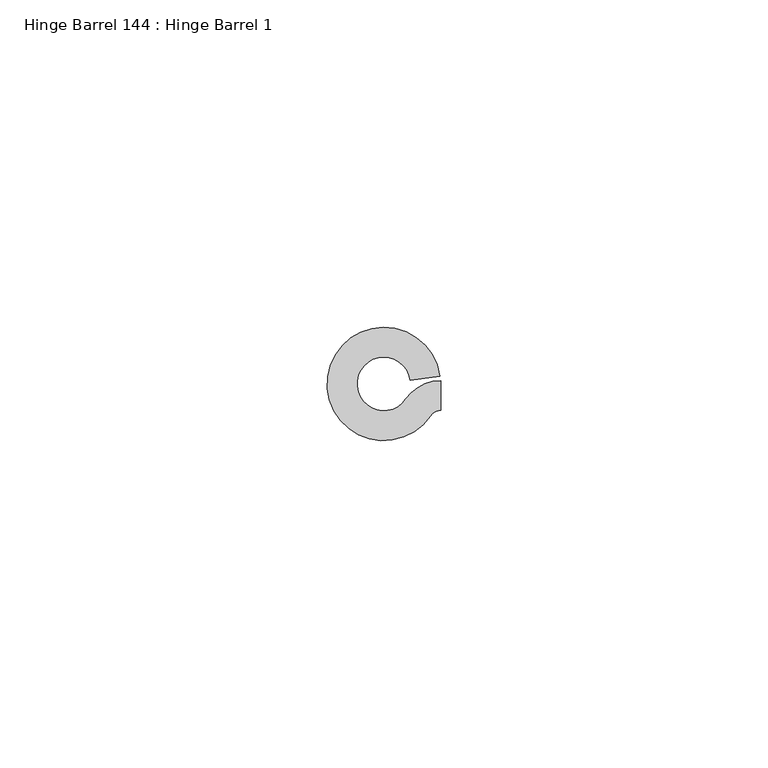
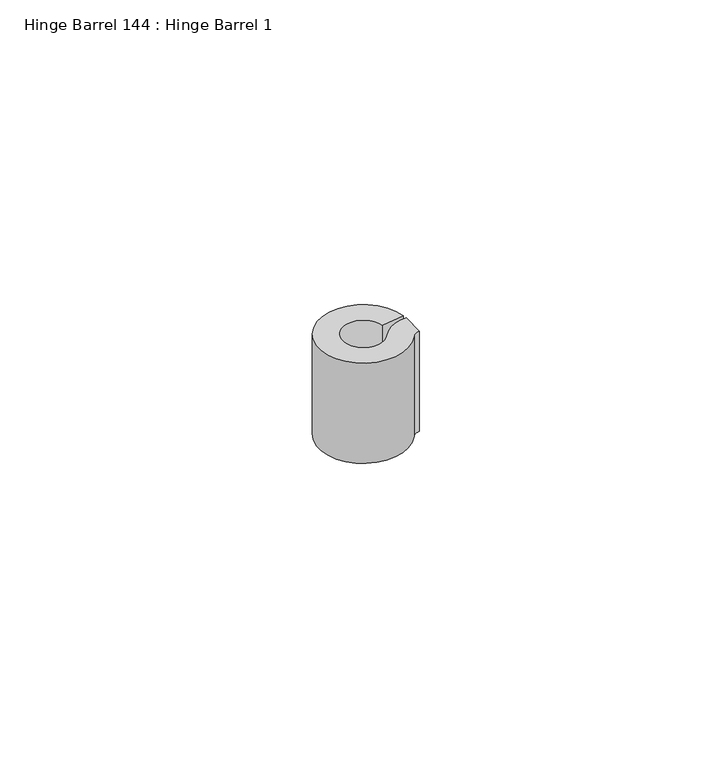
"""IFC4 building model written with IfcOpenShell, lengths in millimetres: proxy geometry, Hinge Barrel 144 : Hinge Barrel 1."""

import ifcopenshell
import ifcopenshell.guid

model = None  # the IFC model being written
_history = None  # IfcOwnerHistory: only IFC2X3 demands one
_inside = {}  # id of a spatial element -> (the spatial element, [elements in it])
_under = {}  # id of a project, library or spatial element -> (it, [spatial elements below it])
_declared = {}  # id of a project -> (the project, [libraries it declares])
_typed = {}  # id of a type object -> (the type object, [elements of that type])
_made_of = {}  # id of a material, layer set ... -> (it, [elements and type objects made of it])


def new_model(schema):
    """Start an empty IFC model of exactly this schema.

    Asked for "IFC4X3", IfcOpenShell would pick the latest addendum, in which some entities
    have other attributes; the version numbers below select the first issue.
    IFC2X3 requires an IfcOwnerHistory on every rooted entity: one is made here for all.
    """
    global model, _history
    if schema == "IFC4X3":
        model = ifcopenshell.file(schema_version=(4, 3, 0, 0))
    else:
        model = ifcopenshell.file(schema=schema)
    _inside.clear()
    _under.clear()
    _declared.clear()
    _typed.clear()
    _made_of.clear()
    _history = None
    if model.schema == "IFC2X3":
        org = make("IfcOrganization", Name="unknown")
        user = make(
            "IfcPersonAndOrganization",
            ThePerson=make("IfcPerson", FamilyName="unknown"),
            TheOrganization=org,
        )
        app = make(
            "IfcApplication",
            ApplicationDeveloper=org,
            Version="unknown",
            ApplicationFullName="unknown",
            ApplicationIdentifier="unknown",
        )
        _history = make(
            "IfcOwnerHistory",
            OwningUser=user,
            OwningApplication=app,
            ChangeAction="ADDED",
            CreationDate=0,
        )
    return model


def make(cls, **values):
    """One entity of the class cls with the attributes given. An attribute that is None is left unset."""
    return model.create_entity(
        cls, **{name: value for name, value in values.items() if value is not None}
    )


def rooted(cls, **values):
    """An entity with a GlobalId (a new one), such as an element, a storey or a relation."""
    return make(cls, GlobalId=ifcopenshell.guid.new(), OwnerHistory=_history, **values)


def si_unit(unit_type, name, prefix=None):
    """IfcSIUnit, for example si_unit("LENGTHUNIT", "METRE", prefix="MILLI")."""
    return make("IfcSIUnit", UnitType=unit_type, Prefix=prefix, Name=name)


def assignment(units):
    """IfcUnitAssignment: the units of a project."""
    return None if units is None else make("IfcUnitAssignment", Units=units)


def point(xyz):
    """IfcCartesianPoint."""
    return None if xyz is None else make("IfcCartesianPoint", Coordinates=xyz)


def direction(xyz):
    """IfcDirection."""
    return None if xyz is None else make("IfcDirection", DirectionRatios=xyz)


def frame(location, z_axis=None, x_axis=None):
    """IfcAxis2Placement3D, a coordinate frame: its origin and axes. An axis left out is left unset."""
    return make(
        "IfcAxis2Placement3D",
        Location=point(location),
        Axis=direction(z_axis),
        RefDirection=direction(x_axis),
    )


def frame_2d(location, x_axis=None):
    """IfcAxis2Placement2D, a coordinate frame in the plane: its origin and x axis."""
    return make(
        "IfcAxis2Placement2D", Location=point(location), RefDirection=direction(x_axis)
    )


def origin():
    """The frame at (0, 0, 0) with its axes left unset."""
    return frame((0.0, 0.0, 0.0))


def place(relative_to, where):
    """IfcLocalPlacement: puts the frame where relative to a parent placement (None: the world)."""
    return make(
        "IfcLocalPlacement", PlacementRelTo=relative_to, RelativePlacement=where
    )


def context(
    kind, dimensions, precision=None, world=None, true_north=None, identifier=None
):
    """IfcGeometricRepresentationContext, for example the 3D "Model" context."""
    return make(
        "IfcGeometricRepresentationContext",
        ContextIdentifier=identifier,
        ContextType=kind,
        CoordinateSpaceDimension=dimensions,
        Precision=precision,
        WorldCoordinateSystem=world,
        TrueNorth=true_north,
    )


def project(units=None, contexts=None):
    """IfcProject with its units and contexts."""
    return rooted(
        "IfcProject",
        Name="project",
        RepresentationContexts=contexts,
        UnitsInContext=assignment(units),
    )


def spatial(cls, under=None, at=None, **own):
    """A site, building, storey or space (cls), placed at a placement, below another one or the project."""
    s = rooted(cls, ObjectPlacement=at, **own)
    if under is not None:
        _under.setdefault(under.id(), (under, []))[1].append(s)
    return s


def polyline(points):
    """IfcPolyline through the points."""
    return make("IfcPolyline", Points=[point(p) for p in points])


def circle_curve(where, radius):
    """IfcCircle in the frame where."""
    return make("IfcCircle", Position=where, Radius=radius)


def trimmed(basis, trim1, trim2, sense, master):
    """IfcTrimmedCurve: the piece of a basis curve between two trims."""
    return make(
        "IfcTrimmedCurve",
        BasisCurve=basis,
        Trim1=trim1,
        Trim2=trim2,
        SenseAgreement=sense,
        MasterRepresentation=master,
    )


def segment(curve, same_sense, transition):
    """IfcCompositeCurveSegment."""
    return make(
        "IfcCompositeCurveSegment",
        Transition=transition,
        SameSense=same_sense,
        ParentCurve=curve,
    )


def composite_curve(segments, self_intersect=None):
    """IfcCompositeCurve: segments joined end to end."""
    return make("IfcCompositeCurve", Segments=segments, SelfIntersect=self_intersect)


def outline(outer, holes=None, kind="AREA"):
    """IfcArbitraryClosedProfileDef: a profile drawn as a closed curve; with holes, ...WithVoids."""
    if holes is None:
        return make("IfcArbitraryClosedProfileDef", ProfileType=kind, OuterCurve=outer)
    return make(
        "IfcArbitraryProfileDefWithVoids",
        ProfileType=kind,
        OuterCurve=outer,
        InnerCurves=holes,
    )


def extrude(swept, where, along, depth):
    """IfcExtrudedAreaSolid: the profile swept, set in the frame where, extruded along a direction by depth."""
    return make(
        "IfcExtrudedAreaSolid",
        SweptArea=swept,
        Position=where,
        ExtrudedDirection=direction(along),
        Depth=depth,
    )


def shape(context_of_items, identifier, shape_type, items):
    """IfcShapeRepresentation: the items that make up one representation, for example the "Body"."""
    return make(
        "IfcShapeRepresentation",
        ContextOfItems=context_of_items,
        RepresentationIdentifier=identifier,
        RepresentationType=shape_type,
        Items=items,
    )


def source(mapping_origin, context_of_items, identifier, shape_type, items):
    """IfcRepresentationMap: a shape defined once, which mapped items show again and again."""
    return make(
        "IfcRepresentationMap",
        MappingOrigin=mapping_origin,
        MappedRepresentation=shape(context_of_items, identifier, shape_type, items),
    )


def transform(
    local_origin,
    x_axis=None,
    y_axis=None,
    z_axis=None,
    scale=None,
    scale2=None,
    scale3=None,
    uniform=True,
):
    """IfcCartesianTransformationOperator3D, or its non-uniform kind. x_axis, y_axis, z_axis: its Axis1, 2, 3."""
    if uniform:
        return make(
            "IfcCartesianTransformationOperator3D",
            Axis1=direction(x_axis),
            Axis2=direction(y_axis),
            LocalOrigin=point(local_origin),
            Scale=scale,
            Axis3=direction(z_axis),
        )
    return make(
        "IfcCartesianTransformationOperator3DnonUniform",
        Axis1=direction(x_axis),
        Axis2=direction(y_axis),
        LocalOrigin=point(local_origin),
        Scale=scale,
        Axis3=direction(z_axis),
        Scale2=scale2,
        Scale3=scale3,
    )


def mapped(mapping_source, mapping_target):
    """IfcMappedItem: shows the shape of a source again, moved by a transform."""
    return make(
        "IfcMappedItem", MappingSource=mapping_source, MappingTarget=mapping_target
    )


def made_of(thing, what):
    """Note that an element or type object is made of a material, layer set ...; save() writes the relation."""
    if what is not None:
        _made_of.setdefault(what.id(), (what, []))[1].append(thing)
    return thing


def element(
    cls,
    number,
    at=None,
    inside=None,
    cuts=None,
    type_object=None,
    material=None,
    context=None,
    identifier="Body",
    shape_type=None,
    held_by="IfcProductDefinitionShape",
    body=None,
    shapes=None,
    **own,
):
    """One element of the class cls, such as IfcWall. Its Tag is "e" and its number.

    at: its placement. inside: the storey or other place that contains it. cuts: it is an
    opening in that element (IfcRelVoidsElement). A single representation is given by context,
    identifier, shape_type and body (its items); several are given by shapes. held_by: the class
    of the entity that holds the representations. save() writes the other relations.
    """
    e = rooted(cls, Tag="e%d" % number, ObjectPlacement=at, **own)
    if body is not None:
        shapes = [shape(context, identifier, shape_type, body)]
    if shapes is not None:
        e.Representation = make(held_by, Representations=shapes)
    if inside is not None:
        _inside.setdefault(inside.id(), (inside, []))[1].append(e)
    if cuts is not None:
        rooted(
            "IfcRelVoidsElement", RelatingBuildingElement=cuts, RelatedOpeningElement=e
        )
    if type_object is not None:
        _typed.setdefault(type_object.id(), (type_object, []))[1].append(e)
    return made_of(e, material)


def aggregate(whole, parts):
    """IfcRelAggregates: a whole, such as a stair, and the parts it consists of."""
    return rooted("IfcRelAggregates", RelatingObject=whole, RelatedObjects=parts)


def save(model, path):
    """Write the relations noted so far, then the file.

    IfcRelAggregates (storeys below a building ...), IfcRelContainedInSpatialStructure (elements
    in a storey), IfcRelDefinesByType, IfcRelAssociatesMaterial and IfcRelDeclares: one each for
    every whole, place, type object, material and project.
    """
    for whole, parts in _under.values():
        aggregate(whole, parts)
    for where, things in _inside.values():
        rooted(
            "IfcRelContainedInSpatialStructure",
            RelatedElements=things,
            RelatingStructure=where,
        )
    for kind, things in _typed.values():
        rooted("IfcRelDefinesByType", RelatedObjects=things, RelatingType=kind)
    for what, things in _made_of.values():
        rooted("IfcRelAssociatesMaterial", RelatedObjects=things, RelatingMaterial=what)
    for by, libraries in _declared.values():
        rooted("IfcRelDeclares", RelatingContext=by, RelatedDefinitions=libraries)
    model.write(path)


def hinge_barrel_144_hinge_barrel_1_f5069254(model_context):
    return source(origin(), model_context, "Body", "SweptSolid", [
        extrude(outline(composite_curve([segment(trimmed(circle_curve(frame_2d((587327.8245257, -536316.2443067)), 6.4044851), [point((587322.5194669, -536312.6563017))], [point((587327.8245257, -536309.8398216))], False, "CARTESIAN"), True, "CONTINUOUS"), segment(polyline([(587327.8245257, -536309.8398216), (587327.8245257, -536314.4038841)]), True, "CONTINUOUS"), segment(trimmed(circle_curve(frame_2d((587327.8245257, -536316.2443067)), 1.8404226), [point((587327.8245257, -536314.4038841))], [point((587326.3000393, -536315.2132409))], True, "CARTESIAN"), True, "CONTINUOUS"), segment(trimmed(circle_curve(frame_2d((587319.1320739, -536310.3652841)), 8.6534625), [point((587326.3000393, -536315.2132409))], [point((587327.7022899, -536309.1678654))], False, "CARTESIAN"), True, "CONTINUOUS"), segment(polyline([(587327.7022899, -536309.1678654), (587323.1821338, -536309.7994153)]), True, "CONTINUOUS"), segment(trimmed(circle_curve(frame_2d((587319.1320739, -536310.3652841)), 4.0894), [point((587323.1821338, -536309.7994153))], [point((587322.5194669, -536312.6563017))], True, "CARTESIAN"), True, "CONTINUOUS")], self_intersect=False)), frame((0.0, 0.0, 1250.95), z_axis=(0.0, 0.0, 1.0), x_axis=(1.0, 0.0, 0.0)), (0.0, 0.0, 1.0), 20.8359375),
    ])


if __name__ == "__main__":
    model = new_model("IFC4")
    model_context = context("Model", 3, world=origin())
    ifc_project = project(units=[si_unit("LENGTHUNIT", "METRE", prefix="MILLI")], contexts=[model_context])
    site = spatial("IfcSite", under=ifc_project)
    building = spatial("IfcBuilding", under=site)
    placement = place(None, origin())
    hinge_barrel_144_hinge_barrel_1_shape = hinge_barrel_144_hinge_barrel_1_f5069254(model_context)
    element("IfcBuildingElementProxy", 1, Name="Hinge Barrel 144 : Hinge Barrel 1", ObjectType="Hinge Barrel 144 : Hinge Barrel 1", at=placement, inside=building, context=model_context, shape_type="MappedRepresentation", body=[
        mapped(hinge_barrel_144_hinge_barrel_1_shape, transform((0.0, 0.0, 0.0), x_axis=(1.0, 0.0, 0.0), y_axis=(0.0, 1.0, 0.0), z_axis=(0.0, 0.0, 1.0))),
    ])
    save(model, "model.ifc")

# Revit data of these elements
# Element 1 (IfcBuildingElementProxy, "Hinge Barrel 144 : Hinge Barrel 1")
#   Materials on its faces: "6\"X6\" WELD-ON STL BUTT HINGE"
# Materials
#   "6\"X6\" WELD-ON STL BUTT HINGE": class "Metal", colour RGB 189 187 185, transparency 0, Description = "Carbon steel", Cost = 0
